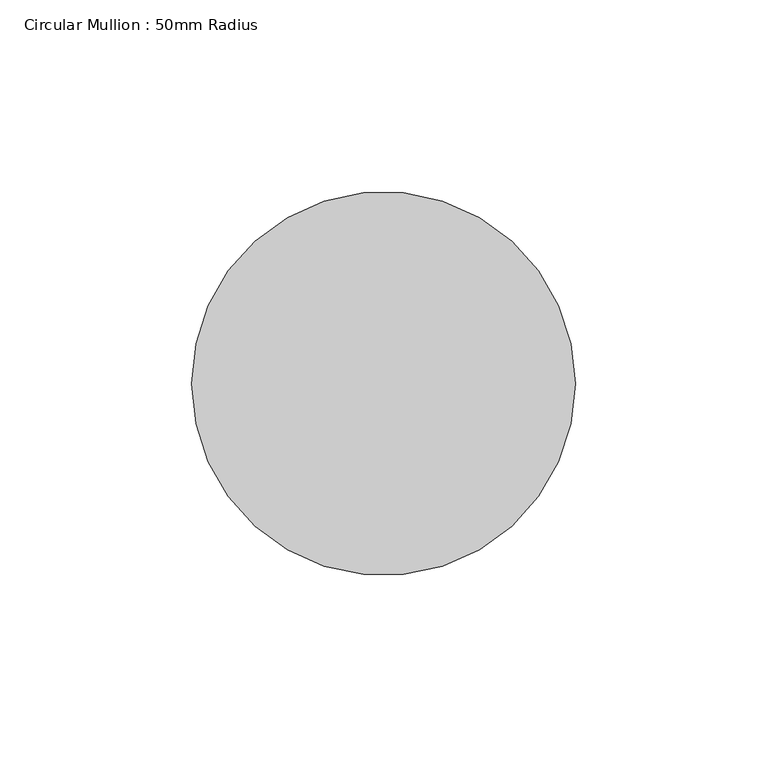
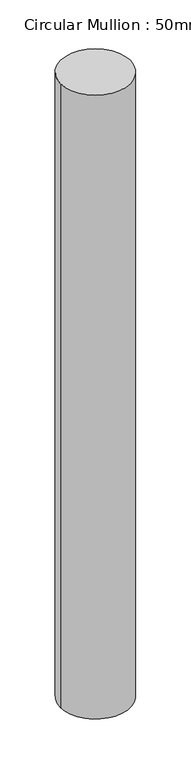
"""IFC4 building model written with IfcOpenShell, lengths in millimetres: member geometry, Circular Mullion : 50mm Radius."""

from ifc_helpers import new_model, si_unit, point, frame, origin, origin_2d, place, context, project, spatial, circle_curve, trimmed, segment, composite_curve, outline, extrude, source, transform, mapped, element, save


def circular_mullion_50mm_radius_5f64c23d(model_context):
    return source(origin(), model_context, "Body", "SweptSolid", [
        extrude(outline(composite_curve([segment(trimmed(circle_curve(origin_2d(), 50.0), [point((50.0, 0.0))], [point((-50.0, 0.0))], False, "CARTESIAN"), True, "CONTINUOUS"), segment(trimmed(circle_curve(origin_2d(), 50.0), [point((-50.0, 0.0))], [point((50.0, 0.0))], False, "CARTESIAN"), True, "CONTINUOUS")], self_intersect=False)), frame((0.0, 0.0, -942.7718173), z_axis=(0.0, 0.0, 1.0), x_axis=(1.0, 0.0, 0.0)), (0.0, 0.0, 1.0), 942.7718173),
    ])


if __name__ == "__main__":
    model = new_model("IFC4")
    model_context = context("Model", 3, world=origin())
    ifc_project = project(units=[si_unit("LENGTHUNIT", "METRE", prefix="MILLI")], contexts=[model_context])
    site = spatial("IfcSite", under=ifc_project)
    building = spatial("IfcBuilding", under=site)
    placement = place(None, origin())
    circular_mullion_50mm_radius_shape = circular_mullion_50mm_radius_5f64c23d(model_context)
    element("IfcMember", 1, ObjectType="Circular Mullion : 50mm Radius", at=placement, inside=building, context=model_context, shape_type="MappedRepresentation", body=[
        mapped(circular_mullion_50mm_radius_shape, transform((0.0, 0.0, 0.0), x_axis=(1.0, 0.0, 0.0), y_axis=(0.0, 1.0, 0.0), z_axis=(0.0, 0.0, 1.0))),
    ])
    save(model, "model.ifc")

# Revit data of these elements
# Type "Circular Mullion : 50mm Radius"
#   built-in parameter 1007350 = 0.164042 (stored number, unit not read)
# Element 1 (IfcMember, "Circular Mullion : 50mm Radius")
#   Materials on its faces: "Aluminium"
# Materials
#   "Aluminium": class "Metal", colour RGB 247 247 247, transparency 0, Description = "Aluminium 6061", Cost = 0
